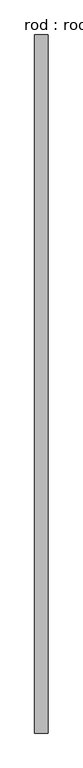
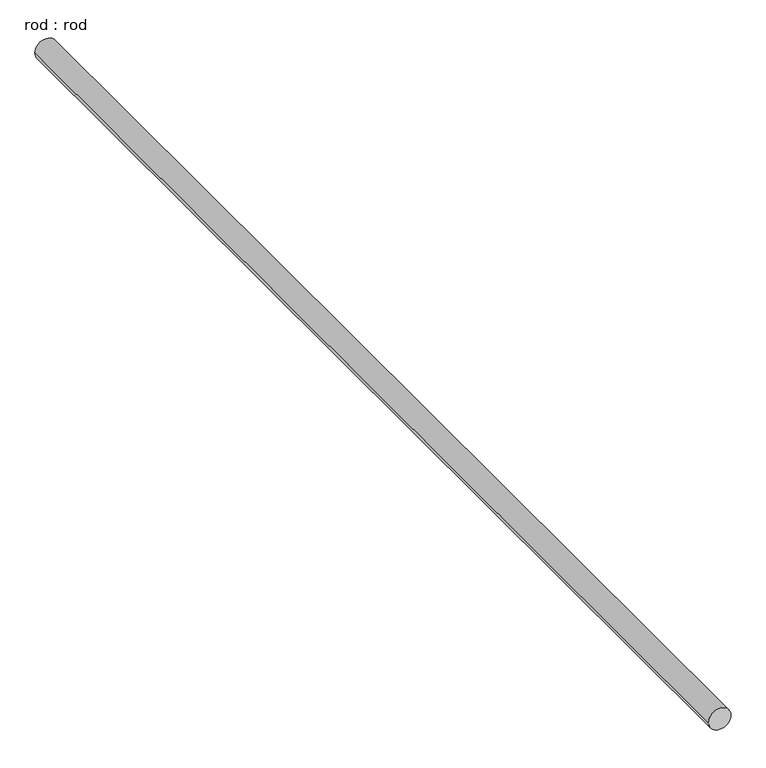
"""IFC4 building model written with IfcOpenShell, lengths in millimetres: proxy geometry, rod : rod."""

from ifc_helpers import new_model, si_unit, point, frame, frame_2d, origin, place, context, project, spatial, circle_curve, trimmed, segment, composite_curve, outline, extrude, source, transform, mapped, element, save


def rod_rod_7d27799d(model_context):
    return source(origin(), model_context, "Body", "SweptSolid", [
        extrude(outline(composite_curve([segment(trimmed(circle_curve(frame_2d((0.0108462, 0.0)), 200.0), [point((0.0108462, 200.0))], [point((0.0108462, -200.0))], False, "CARTESIAN"), True, "CONTINUOUS"), segment(trimmed(circle_curve(frame_2d((0.0108462, 0.0)), 200.0), [point((0.0108462, -200.0))], [point((0.0108462, 200.0))], False, "CARTESIAN"), True, "CONTINUOUS")], self_intersect=False)), frame((0.0, -6340.3070989, 0.0), z_axis=(0.0, 1.0, 0.0), x_axis=(0.0, 0.0, 1.0)), (0.0, 0.0, 1.0), 20866.0714286),
    ])


if __name__ == "__main__":
    model = new_model("IFC4")
    model_context = context("Model", 3, world=origin())
    ifc_project = project(units=[si_unit("LENGTHUNIT", "METRE", prefix="MILLI")], contexts=[model_context])
    site = spatial("IfcSite", under=ifc_project)
    building = spatial("IfcBuilding", under=site)
    placement = place(None, origin())
    rod_rod_shape = rod_rod_7d27799d(model_context)
    element("IfcBuildingElementProxy", 1, Name="rod : rod", ObjectType="rod : rod", at=placement, inside=building, context=model_context, shape_type="MappedRepresentation", body=[
        mapped(rod_rod_shape, transform((0.0, 0.0, 0.0), x_axis=(1.0, 0.0, 0.0), y_axis=(0.0, 1.0, 0.0), z_axis=(0.0, 0.0, 1.0))),
    ])
    save(model, "model.ifc")

# Revit data of these elements
# Type "rod : rod"
#   Default Elevation = 0
